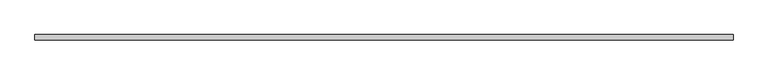
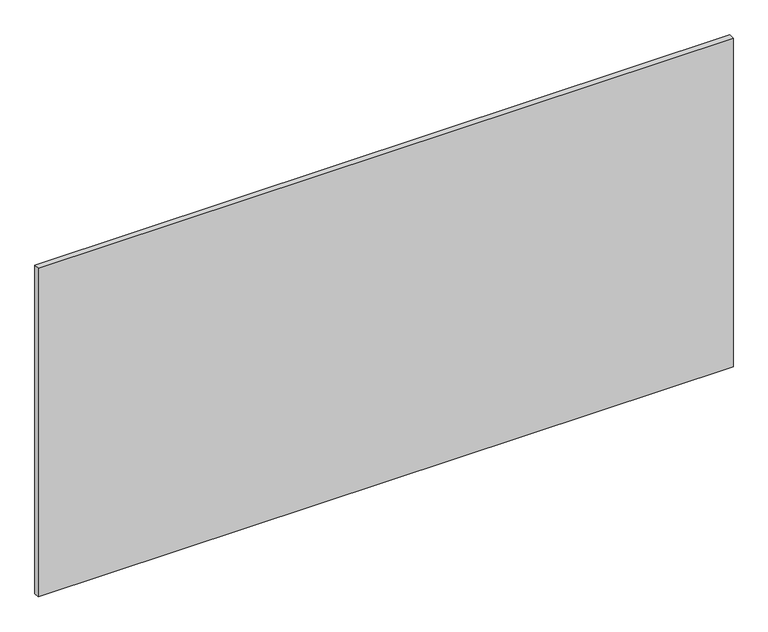
"""IFC4 building model written with IfcOpenShell, lengths in millimetres: proxy geometry, Inner panel:Inner panel:1:Inner panel:1 : Inner panel:Inner panel:300324:300043:Inner panel:1:Inner panel:1 : Inner panel:Inner panel:300324:300043 : Inner panel:Inner panel:1:Inner panel:1 : Inner panel:Inner panel:300324:300043:1 : Inner panel:Inner panel:1:Inner panel:1 : Inner panel:Inner panel:300324:300043:Inner panel:1:Inner panel:1 : Inner panel:Inner panel:300324:300043 : Inner panel:Inner panel:1:Inner panel:1 : Inner panel:Inner panel:300324:300043:300031."""

from ifc_helpers import new_model, si_unit, frame, origin, place, context, project, spatial, polyline, outline, extrude, source, transform, mapped, element, save


def generic_models_61a3d693(model_context):
    return source(origin(), model_context, "Body", "SweptSolid", [
        extrude(outline(polyline([(593738.0867239, -578778.4413841), (596176.4867239, -578778.4413841), (596176.4867239, -578797.4913841), (593738.0867239, -578797.4913841), (593738.0867239, -578778.4413841)])), frame((0.0, 0.0, 44.45), z_axis=(0.0, 0.0, 1.0), x_axis=(1.0, 0.0, 0.0)), (0.0, 0.0, 1.0), 1219.2),
    ])


if __name__ == "__main__":
    model = new_model("IFC4")
    model_context = context("Model", 3, world=origin())
    ifc_project = project(units=[si_unit("LENGTHUNIT", "METRE", prefix="MILLI")], contexts=[model_context])
    site = spatial("IfcSite", under=ifc_project)
    building = spatial("IfcBuilding", under=site)
    placement = place(None, origin())
    generic_models_shape = generic_models_61a3d693(model_context)
    element("IfcBuildingElementProxy", 1, Name="Inner panel:Inner panel:1:Inner panel:1 : Inner panel:Inner panel:300324:300043:Inner panel:1:Inner panel:1 : Inner panel:Inner panel:300324:300043 : Inner panel:Inner panel:1:Inner panel:1 : Inner panel:Inner panel:300324:300043:1 : Inner panel:Inner panel:1:Inner panel:1 : Inner panel:Inner panel:300324:300043:Inner panel:1:Inner panel:1 : Inner panel:Inner panel:300324:300043 : Inner panel:Inner panel:1:Inner panel:1 : Inner panel:Inner panel:300324:300043:300031", ObjectType="Inner panel:Inner panel:1:Inner panel:1 : Inner panel:Inner panel:300324:300043:Inner panel:1:Inner panel:1 : Inner panel:Inner panel:300324:300043 : Inner panel:Inner panel:1:Inner panel:1 : Inner panel:Inner panel:300324:300043:1 : Inner panel:Inner panel:1:Inner panel:1 : Inner panel:Inner panel:300324:300043:Inner panel:1:Inner panel:1 : Inner panel:Inner panel:300324:300043 : Inner panel:Inner panel:1:Inner panel:1 : Inner panel:Inner panel:300324:300043:300031", at=placement, inside=building, context=model_context, shape_type="MappedRepresentation", body=[
        mapped(generic_models_shape, transform((0.0, 0.0, 0.0), x_axis=(1.0, 0.0, 0.0), y_axis=(0.0, 1.0, 0.0), z_axis=(0.0, 0.0, 1.0))),
    ])
    save(model, "model.ifc")

# Revit data of these elements
# Type "Inner panel:Inner panel:1:Inner panel:1 : Inner panel:Inner panel:300324:300043:Inner panel:1:Inner panel:1 : Inner panel:Inner panel:300324:300043 : Inner panel:Inner panel:1:Inner panel:1 : Inner panel:Inner panel:300324:300043:1 : Inner panel:Inner panel:1:Inner panel:1 : Inner panel:Inner panel:300324:300043:Inner panel:1:Inner panel:1 : Inner panel:Inner panel:300324:300043 : Inner panel:Inner panel:1:Inner panel:1 : Inner panel:Inner panel:300324:300043:300031"
#   NameOverride = "Inner panel:Inner panel:1:Inner panel:1 : Inner panel:Inner panel:300324:300043:Inner panel:1:Inner panel:1 : Inner panel:Inner panel:300324:300043 : Inner panel:Inner panel:1:Inner panel:1 : Inner panel:Inner panel:300324:300043:300031"
#   ObjectTypeOverride = "Inner panel:1:Inner panel:1 : Inner panel:Inner panel:300324:300043 : Inner panel:Inner panel:1:Inner panel:1 : Inner panel:Inner panel:300324:300043"
#   Reference = "Inner panel"
#   Tag = "300031"
# Element 1 (IfcBuildingElementProxy, "Inner panel:Inner panel:1:Inner panel:1 : Inner panel:Inner panel:300324:300043:Inner panel:1:Inner panel:1 : Inner panel:Inner panel:300324:300043 : Inner panel:Inner panel:1:Inner panel:1 : Inner panel:Inner panel:300324:300043:1 : Inner panel:Inner panel:1:Inner panel:1 : Inner panel:Inner panel:300324:300043:Inner panel:1:Inner panel:1 : Inner panel:Inner panel:300324:300043 : Inner panel:Inner panel:1:Inner panel:1 : Inner panel:Inner panel:300324:300043:300031")
#   Materials on its faces: "3/4\" PREFINISHED STAINED/SEALED PLYWOOD (FINISH: GRADE B,  FLAME SPREAD: CLASS B)"
# Materials
#   "3/4\" PREFINISHED STAINED/SEALED PLYWOOD (FINISH: GRADE B,  FLAME SPREAD: CLASS B)": class "Wood", colour RGB 149 120 74, transparency 0, Description = "Plywood, sheathing grade", Cost = 0
